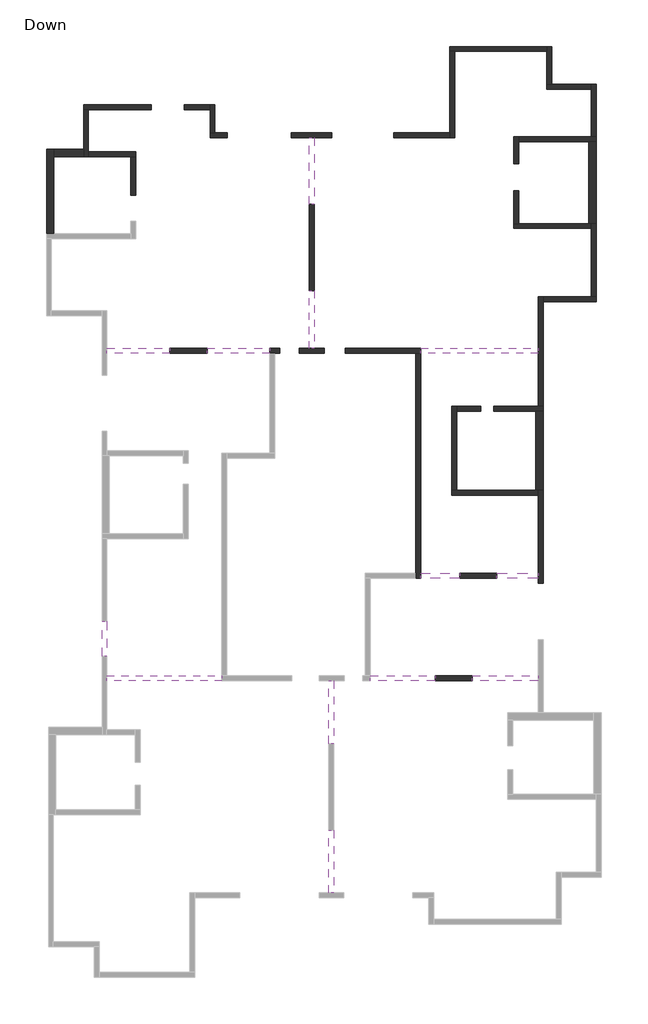
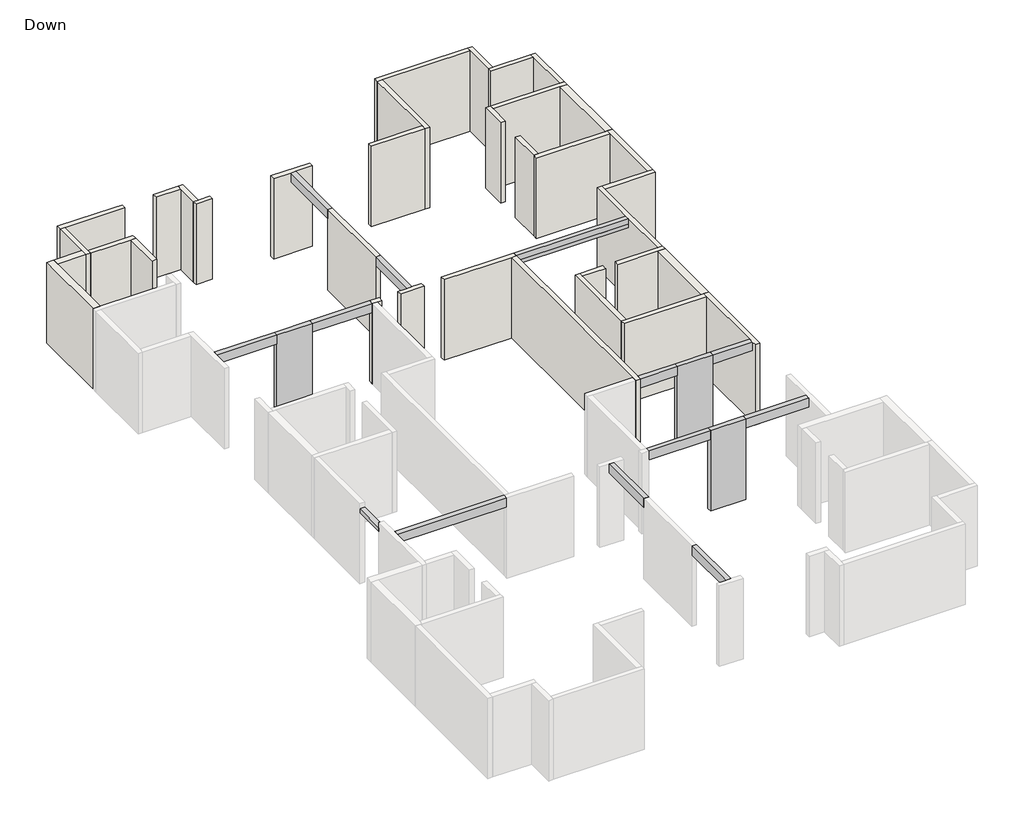
# One storey, part 2 of 2: 35 walls, 13 beams, 3 columns.
# Revit data of these elements (continued)
# Element 39 (IfcWall, "20") (continued)
#   Top Offset = 0 cm
#   Base Offset = 0 cm
#   wall height = 360 cm
#   SOFiSTiK_AMG_Scheduled = yes
#   SOFiSTiK_AMG_Adjusted = yes
#   Phase Created = New Construction
#   Base Constraint = Down
#   Top Constraint = Typical Floor
#   Materials on its faces: "Concrete"
# Element 40 (IfcWall, "20")
#   Comments = ""
#   Mark = "W66"
#   SOFiSTiK_EdgeZones = "W67"
#   SOFiSTiK_AMG_Comments = ""
#   Top Offset = 0 cm
#   Base Offset = 0 cm
#   wall height = 360 cm
#   SOFiSTiK_AMG_Scheduled = yes
#   SOFiSTiK_AMG_Adjusted = yes
#   Phase Created = New Construction
#   Base Constraint = Down
#   Top Constraint = Typical Floor
#   Materials on its faces: "Concrete"
# Element 41 (IfcWall, "20")
#   Comments = ""
#   Mark = "W67"
#   SOFiSTiK_EdgeZones = "W68"
#   SOFiSTiK_AMG_Comments = ""
#   Top Offset = 0 cm
#   Base Offset = 0 cm
#   wall height = 360 cm
#   SOFiSTiK_AMG_Scheduled = yes
#   SOFiSTiK_AMG_Adjusted = yes
#   Phase Created = New Construction
#   Base Constraint = Down
#   Top Constraint = Typical Floor
#   Materials on its faces: "Concrete"
# Element 42 (IfcWall, "20")
#   Comments = ""
#   Mark = "W72"
#   SOFiSTiK_EdgeZones = "W73"
#   SOFiSTiK_AMG_Comments = ""
#   Top Offset = 0 cm
#   Base Offset = 0 cm
#   wall height = 360 cm
#   SOFiSTiK_AMG_Scheduled = yes
#   SOFiSTiK_AMG_Adjusted = yes
#   Phase Created = New Construction
#   Base Constraint = Down
#   Top Constraint = Typical Floor
#   Materials on its faces: "Concrete"
# Element 43 (IfcWall, "20")
#   Comments = ""
#   Mark = "W73"
#   SOFiSTiK_EdgeZones = "W74"
#   SOFiSTiK_AMG_Comments = ""
#   Top Offset = 0 cm
#   Base Offset = 0 cm
#   wall height = 360 cm
#   SOFiSTiK_AMG_Scheduled = yes
#   SOFiSTiK_AMG_Adjusted = yes
#   Phase Created = New Construction
#   Base Constraint = Down
#   Top Constraint = Typical Floor
#   Materials on its faces: "Concrete"
# Element 44 (IfcWall, "20")
#   Comments = ""
#   Mark = "W74"
#   SOFiSTiK_EdgeZones = "W75"
#   SOFiSTiK_AMG_Comments = ""
#   Top Offset = 0 cm
#   Base Offset = 0 cm
#   wall height = 360 cm
#   SOFiSTiK_AMG_Scheduled = yes
#   SOFiSTiK_AMG_Adjusted = yes
#   Phase Created = New Construction
#   Base Constraint = Down
#   Top Constraint = Typical Floor
#   Materials on its faces: "Concrete"
# Element 45 (IfcWall, "20")
#   Comments = ""
#   Mark = "W75"
#   SOFiSTiK_EdgeZones = "W76"
#   SOFiSTiK_AMG_Comments = ""
#   Top Offset = 0 cm
#   Base Offset = 0 cm
#   wall height = 360 cm
#   SOFiSTiK_AMG_Scheduled = yes
#   SOFiSTiK_AMG_Adjusted = yes
#   Phase Created = New Construction
#   Base Constraint = Down
#   Top Constraint = Typical Floor
#   Materials on its faces: "Concrete"
# Element 46 (IfcWall, "20")
#   Comments = ""
#   Mark = "W80"
#   SOFiSTiK_EdgeZones = "W81"
#   SOFiSTiK_AMG_Comments = ""
#   Top Offset = 0 cm
#   Base Offset = 0 cm
#   wall height = 360 cm
#   SOFiSTiK_AMG_Scheduled = yes
#   SOFiSTiK_AMG_Adjusted = yes
#   Phase Created = New Construction
#   Base Constraint = Down
#   Top Constraint = Typical Floor
#   Materials on its faces: "Concrete"
# Element 47 (IfcWall, "20")
#   Comments = ""
#   Mark = "W81"
#   SOFiSTiK_EdgeZones = "W13"
#   SOFiSTiK_AMG_Comments = ""
#   Top Offset = 0 cm
#   Base Offset = 0 cm
#   wall height = 360 cm
#   SOFiSTiK_AMG_Scheduled = yes
#   SOFiSTiK_AMG_Adjusted = yes
#   Phase Created = New Construction
#   Base Constraint = Down
#   Top Constraint = Typical Floor
#   Materials on its faces: "Concrete"
# Element 48 (IfcWall, "30")
#   Comments = ""
#   Mark = "W1"
#   SOFiSTiK_EdgeZones = "W1"
#   SOFiSTiK_AMG_Comments = ""
#   Top Offset = 0 cm
#   Base Offset = 0 cm
#   wall height = 360 cm
#   SOFiSTiK_AMG_Scheduled = yes
#   SOFiSTiK_AMG_Adjusted = yes
#   Phase Created = New Construction
#   Base Constraint = Down
#   Top Constraint = Typical Floor
#   Materials on its faces: "Concrete"
# Element 49 (IfcWall, "30")
#   Comments = ""
#   Mark = "W2"
#   SOFiSTiK_EdgeZones = "W2"
#   SOFiSTiK_AMG_Comments = ""
#   Top Offset = 0 cm
#   Base Offset = 0 cm
#   wall height = 360 cm
#   SOFiSTiK_AMG_Scheduled = yes
#   SOFiSTiK_AMG_Adjusted = yes
#   Phase Created = New Construction
#   Base Constraint = Down
#   Top Constraint = Typical Floor
#   Materials on its faces: "Concrete"
# Element 50 (IfcWall, "30")
#   Comments = ""
#   Mark = "W8"
#   SOFiSTiK_EdgeZones = "W8"
#   SOFiSTiK_AMG_Comments = ""
#   Top Offset = 0 cm
#   Base Offset = 0 cm
#   wall height = 360 cm
#   SOFiSTiK_AMG_Scheduled = yes
#   SOFiSTiK_AMG_Adjusted = yes
#   Phase Created = New Construction
#   Base Constraint = Down
#   Top Constraint = Typical Floor
#   Materials on its faces: "Concrete"
# Element 51 (IfcWall, "30")
#   Comments = ""
#   Mark = "W9"
#   SOFiSTiK_EdgeZones = "W9"
#   SOFiSTiK_AMG_Comments = ""
#   Top Offset = 0 cm
#   Base Offset = 0 cm
#   wall height = 360 cm
#   SOFiSTiK_AMG_Scheduled = yes
#   SOFiSTiK_AMG_Adjusted = yes
#   Phase Created = New Construction
#   Base Constraint = Down
#   Top Constraint = Typical Floor
#   Materials on its faces: "Concrete"
# Materials
#   "Concrete": class "Concrete", colour RGB 192 192 192, transparency 0, Keynote = "01000", Description = "Cast-in-place concrete", Cost = 0
